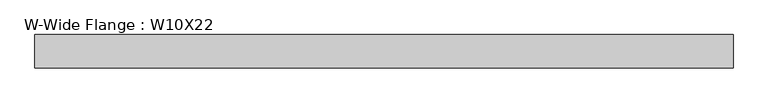
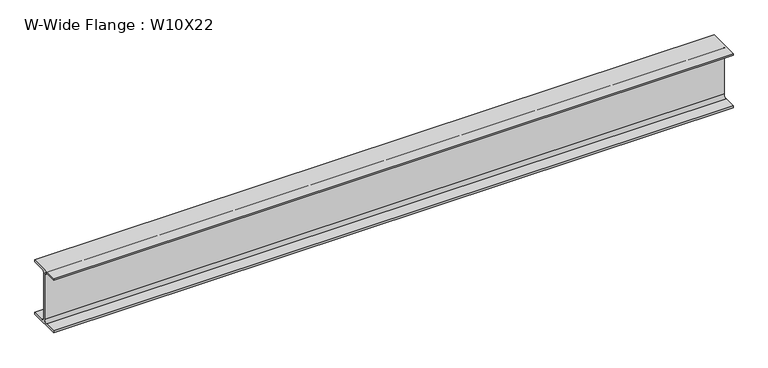
"""IFC4 building model written with IfcOpenShell, lengths in millimetres: beam geometry, W-Wide Flange : W10X22."""

from ifc_helpers import new_model, si_unit, point, frame, frame_2d, origin, place, context, project, spatial, polyline, circle_curve, trimmed, segment, composite_curve, outline, extrude, source, transform, mapped, element, save


def w_wide_flange_w10x22_d9725fee(model_context):
    return source(origin(), model_context, "Body", "SweptSolid", [
        extrude(outline(composite_curve([segment(polyline([(73.025, -120.396), (73.025, -129.54), (-73.025, -129.54), (-73.025, -120.396), (-17.7165, -120.396)]), True, "CONTINUOUS"), segment(trimmed(circle_curve(frame_2d((-17.7165, -105.7275)), 14.6685), [point((-17.7165, -120.396))], [point((-3.048, -105.7275))], True, "CARTESIAN"), True, "CONTINUOUS"), segment(polyline([(-3.048, -105.7275), (-3.048, 105.7275)]), True, "CONTINUOUS"), segment(trimmed(circle_curve(frame_2d((-17.7165, 105.7275)), 14.6685), [point((-3.048, 105.7275))], [point((-17.7165, 120.396))], True, "CARTESIAN"), True, "CONTINUOUS"), segment(polyline([(-17.7165, 120.396), (-73.025, 120.396), (-73.025, 129.54), (73.025, 129.54), (73.025, 120.396), (17.7165, 120.396)]), True, "CONTINUOUS"), segment(trimmed(circle_curve(frame_2d((17.7165, 105.7275)), 14.6685), [point((17.7165, 120.396))], [point((3.048, 105.7275))], True, "CARTESIAN"), True, "CONTINUOUS"), segment(polyline([(3.048, 105.7275), (3.048, -105.7275)]), True, "CONTINUOUS"), segment(trimmed(circle_curve(frame_2d((17.7165, -105.7275)), 14.6685), [point((3.048, -105.7275))], [point((17.7165, -120.396))], True, "CARTESIAN"), True, "CONTINUOUS"), segment(polyline([(17.7165, -120.396), (73.025, -120.396)]), True, "CONTINUOUS")], self_intersect=False)), frame((-1530.35, 0.0, 0.0), z_axis=(1.0, 0.0, 0.0), x_axis=(0.0, 1.0, 0.0)), (0.0, 0.0, 1.0), 3060.7),
    ])


if __name__ == "__main__":
    model = new_model("IFC4")
    model_context = context("Model", 3, world=origin())
    ifc_project = project(units=[si_unit("LENGTHUNIT", "METRE", prefix="MILLI")], contexts=[model_context])
    site = spatial("IfcSite", under=ifc_project)
    building = spatial("IfcBuilding", under=site)
    placement = place(None, origin())
    w_wide_flange_w10x22_shape = w_wide_flange_w10x22_d9725fee(model_context)
    element("IfcBeam", 1, ObjectType="W-Wide Flange : W10X22", at=placement, inside=building, context=model_context, shape_type="MappedRepresentation", body=[
        mapped(w_wide_flange_w10x22_shape, transform((0.0, 0.0, 0.0), x_axis=(1.0, 0.0, 0.0), y_axis=(0.0, 1.0, 0.0), z_axis=(0.0, 0.0, 1.0))),
    ])
    save(model, "model.ifc")

# Revit data of these elements
# Type "W-Wide Flange : W10X22"
#   Assembly Code = "B10"
#   W = 22
#   Length [instance default] = 5' - 0"
#   bf = 0' - 5 3/4"
#   d = 0' - 10.2"
#   k = 0' - 0 15/16"
#   k2 = 0' - 0.5775"
#   tf = 0' - 0.36"
#   tw = 0' - 0.24"
#   A = 0.0450694 SF
#   Structural Material [instance default] = _STRUCTURAL STEEL (SEE STRUCT. DWGS)
# Element 1 (IfcBeam, "W-Wide Flange : W10X22")
#   Materials on its faces: "_STRUCTURAL STEEL (SEE STRUCT. DWGS)"
# Materials
#   "_STRUCTURAL STEEL (SEE STRUCT. DWGS)": class "Metal", colour RGB 199 199 199, transparency 0, Description = "Structural steel 50ksi", Cost = 0
